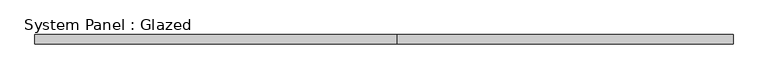
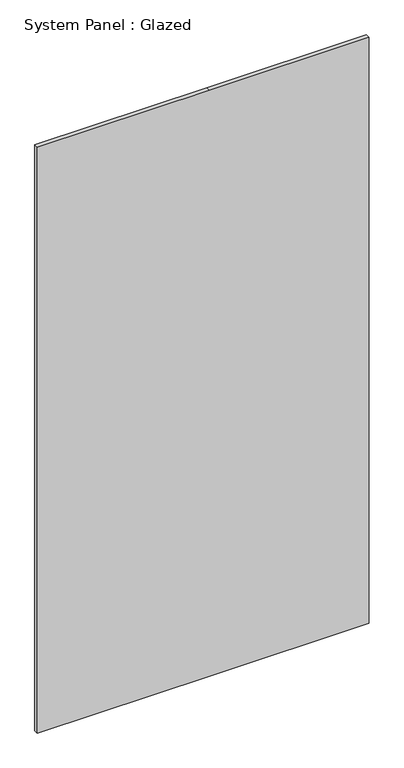
"""IFC4 building model written with IfcOpenShell, lengths in millimetres: plate geometry, System Panel : Glazed."""

import ifcopenshell
import ifcopenshell.guid

model = None  # the IFC model being written
_history = None  # IfcOwnerHistory: only IFC2X3 demands one
_inside = {}  # id of a spatial element -> (the spatial element, [elements in it])
_under = {}  # id of a project, library or spatial element -> (it, [spatial elements below it])
_declared = {}  # id of a project -> (the project, [libraries it declares])
_typed = {}  # id of a type object -> (the type object, [elements of that type])
_made_of = {}  # id of a material, layer set ... -> (it, [elements and type objects made of it])


def new_model(schema):
    """Start an empty IFC model of exactly this schema.

    Asked for "IFC4X3", IfcOpenShell would pick the latest addendum, in which some entities
    have other attributes; the version numbers below select the first issue.
    IFC2X3 requires an IfcOwnerHistory on every rooted entity: one is made here for all.
    """
    global model, _history
    if schema == "IFC4X3":
        model = ifcopenshell.file(schema_version=(4, 3, 0, 0))
    else:
        model = ifcopenshell.file(schema=schema)
    _inside.clear()
    _under.clear()
    _declared.clear()
    _typed.clear()
    _made_of.clear()
    _history = None
    if model.schema == "IFC2X3":
        org = make("IfcOrganization", Name="unknown")
        user = make(
            "IfcPersonAndOrganization",
            ThePerson=make("IfcPerson", FamilyName="unknown"),
            TheOrganization=org,
        )
        app = make(
            "IfcApplication",
            ApplicationDeveloper=org,
            Version="unknown",
            ApplicationFullName="unknown",
            ApplicationIdentifier="unknown",
        )
        _history = make(
            "IfcOwnerHistory",
            OwningUser=user,
            OwningApplication=app,
            ChangeAction="ADDED",
            CreationDate=0,
        )
    return model


def make(cls, **values):
    """One entity of the class cls with the attributes given. An attribute that is None is left unset."""
    return model.create_entity(
        cls, **{name: value for name, value in values.items() if value is not None}
    )


def rooted(cls, **values):
    """An entity with a GlobalId (a new one), such as an element, a storey or a relation."""
    return make(cls, GlobalId=ifcopenshell.guid.new(), OwnerHistory=_history, **values)


def si_unit(unit_type, name, prefix=None):
    """IfcSIUnit, for example si_unit("LENGTHUNIT", "METRE", prefix="MILLI")."""
    return make("IfcSIUnit", UnitType=unit_type, Prefix=prefix, Name=name)


def assignment(units):
    """IfcUnitAssignment: the units of a project."""
    return None if units is None else make("IfcUnitAssignment", Units=units)


def point(xyz):
    """IfcCartesianPoint."""
    return None if xyz is None else make("IfcCartesianPoint", Coordinates=xyz)


def direction(xyz):
    """IfcDirection."""
    return None if xyz is None else make("IfcDirection", DirectionRatios=xyz)


def frame(location, z_axis=None, x_axis=None):
    """IfcAxis2Placement3D, a coordinate frame: its origin and axes. An axis left out is left unset."""
    return make(
        "IfcAxis2Placement3D",
        Location=point(location),
        Axis=direction(z_axis),
        RefDirection=direction(x_axis),
    )


def origin():
    """The frame at (0, 0, 0) with its axes left unset."""
    return frame((0.0, 0.0, 0.0))


def place(relative_to, where):
    """IfcLocalPlacement: puts the frame where relative to a parent placement (None: the world)."""
    return make(
        "IfcLocalPlacement", PlacementRelTo=relative_to, RelativePlacement=where
    )


def context(
    kind, dimensions, precision=None, world=None, true_north=None, identifier=None
):
    """IfcGeometricRepresentationContext, for example the 3D "Model" context."""
    return make(
        "IfcGeometricRepresentationContext",
        ContextIdentifier=identifier,
        ContextType=kind,
        CoordinateSpaceDimension=dimensions,
        Precision=precision,
        WorldCoordinateSystem=world,
        TrueNorth=true_north,
    )


def project(units=None, contexts=None):
    """IfcProject with its units and contexts."""
    return rooted(
        "IfcProject",
        Name="project",
        RepresentationContexts=contexts,
        UnitsInContext=assignment(units),
    )


def spatial(cls, under=None, at=None, **own):
    """A site, building, storey or space (cls), placed at a placement, below another one or the project."""
    s = rooted(cls, ObjectPlacement=at, **own)
    if under is not None:
        _under.setdefault(under.id(), (under, []))[1].append(s)
    return s


def polyline(points):
    """IfcPolyline through the points."""
    return make("IfcPolyline", Points=[point(p) for p in points])


def outline(outer, holes=None, kind="AREA"):
    """IfcArbitraryClosedProfileDef: a profile drawn as a closed curve; with holes, ...WithVoids."""
    if holes is None:
        return make("IfcArbitraryClosedProfileDef", ProfileType=kind, OuterCurve=outer)
    return make(
        "IfcArbitraryProfileDefWithVoids",
        ProfileType=kind,
        OuterCurve=outer,
        InnerCurves=holes,
    )


def extrude(swept, where, along, depth):
    """IfcExtrudedAreaSolid: the profile swept, set in the frame where, extruded along a direction by depth."""
    return make(
        "IfcExtrudedAreaSolid",
        SweptArea=swept,
        Position=where,
        ExtrudedDirection=direction(along),
        Depth=depth,
    )


def shape(context_of_items, identifier, shape_type, items):
    """IfcShapeRepresentation: the items that make up one representation, for example the "Body"."""
    return make(
        "IfcShapeRepresentation",
        ContextOfItems=context_of_items,
        RepresentationIdentifier=identifier,
        RepresentationType=shape_type,
        Items=items,
    )


def source(mapping_origin, context_of_items, identifier, shape_type, items):
    """IfcRepresentationMap: a shape defined once, which mapped items show again and again."""
    return make(
        "IfcRepresentationMap",
        MappingOrigin=mapping_origin,
        MappedRepresentation=shape(context_of_items, identifier, shape_type, items),
    )


def transform(
    local_origin,
    x_axis=None,
    y_axis=None,
    z_axis=None,
    scale=None,
    scale2=None,
    scale3=None,
    uniform=True,
):
    """IfcCartesianTransformationOperator3D, or its non-uniform kind. x_axis, y_axis, z_axis: its Axis1, 2, 3."""
    if uniform:
        return make(
            "IfcCartesianTransformationOperator3D",
            Axis1=direction(x_axis),
            Axis2=direction(y_axis),
            LocalOrigin=point(local_origin),
            Scale=scale,
            Axis3=direction(z_axis),
        )
    return make(
        "IfcCartesianTransformationOperator3DnonUniform",
        Axis1=direction(x_axis),
        Axis2=direction(y_axis),
        LocalOrigin=point(local_origin),
        Scale=scale,
        Axis3=direction(z_axis),
        Scale2=scale2,
        Scale3=scale3,
    )


def mapped(mapping_source, mapping_target):
    """IfcMappedItem: shows the shape of a source again, moved by a transform."""
    return make(
        "IfcMappedItem", MappingSource=mapping_source, MappingTarget=mapping_target
    )


def made_of(thing, what):
    """Note that an element or type object is made of a material, layer set ...; save() writes the relation."""
    if what is not None:
        _made_of.setdefault(what.id(), (what, []))[1].append(thing)
    return thing


def element(
    cls,
    number,
    at=None,
    inside=None,
    cuts=None,
    type_object=None,
    material=None,
    context=None,
    identifier="Body",
    shape_type=None,
    held_by="IfcProductDefinitionShape",
    body=None,
    shapes=None,
    **own,
):
    """One element of the class cls, such as IfcWall. Its Tag is "e" and its number.

    at: its placement. inside: the storey or other place that contains it. cuts: it is an
    opening in that element (IfcRelVoidsElement). A single representation is given by context,
    identifier, shape_type and body (its items); several are given by shapes. held_by: the class
    of the entity that holds the representations. save() writes the other relations.
    """
    e = rooted(cls, Tag="e%d" % number, ObjectPlacement=at, **own)
    if body is not None:
        shapes = [shape(context, identifier, shape_type, body)]
    if shapes is not None:
        e.Representation = make(held_by, Representations=shapes)
    if inside is not None:
        _inside.setdefault(inside.id(), (inside, []))[1].append(e)
    if cuts is not None:
        rooted(
            "IfcRelVoidsElement", RelatingBuildingElement=cuts, RelatedOpeningElement=e
        )
    if type_object is not None:
        _typed.setdefault(type_object.id(), (type_object, []))[1].append(e)
    return made_of(e, material)


def aggregate(whole, parts):
    """IfcRelAggregates: a whole, such as a stair, and the parts it consists of."""
    return rooted("IfcRelAggregates", RelatingObject=whole, RelatedObjects=parts)


def save(model, path):
    """Write the relations noted so far, then the file.

    IfcRelAggregates (storeys below a building ...), IfcRelContainedInSpatialStructure (elements
    in a storey), IfcRelDefinesByType, IfcRelAssociatesMaterial and IfcRelDeclares: one each for
    every whole, place, type object, material and project.
    """
    for whole, parts in _under.values():
        aggregate(whole, parts)
    for where, things in _inside.values():
        rooted(
            "IfcRelContainedInSpatialStructure",
            RelatedElements=things,
            RelatingStructure=where,
        )
    for kind, things in _typed.values():
        rooted("IfcRelDefinesByType", RelatedObjects=things, RelatingType=kind)
    for what, things in _made_of.values():
        rooted("IfcRelAssociatesMaterial", RelatedObjects=things, RelatingMaterial=what)
    for by, libraries in _declared.values():
        rooted("IfcRelDeclares", RelatingContext=by, RelatedDefinitions=libraries)
    model.write(path)


def system_panel_glazed_5e1ca041(model_context):
    return source(origin(), model_context, "Body", "SweptSolid", [
        extrude(outline(polyline([(0.0, -971.55), (0.0, 37.0416667), (0.0, 971.55), (3625.85, 971.55), (3625.85, 37.0416667), (3625.85, -971.55), (0.0, -971.55)])), frame((0.0, -44.45, 0.0), z_axis=(0.0, 1.0, 0.0), x_axis=(0.0, 0.0, 1.0)), (0.0, 0.0, 1.0), 25.4),
    ])


if __name__ == "__main__":
    model = new_model("IFC4")
    model_context = context("Model", 3, world=origin())
    ifc_project = project(units=[si_unit("LENGTHUNIT", "METRE", prefix="MILLI")], contexts=[model_context])
    site = spatial("IfcSite", under=ifc_project)
    building = spatial("IfcBuilding", under=site)
    placement = place(None, origin())
    system_panel_glazed_shape = system_panel_glazed_5e1ca041(model_context)
    element("IfcPlate", 1, ObjectType="System Panel : Glazed", at=placement, inside=building, context=model_context, shape_type="MappedRepresentation", body=[
        mapped(system_panel_glazed_shape, transform((0.0, 0.0, 0.0), x_axis=(1.0, 0.0, 0.0), y_axis=(0.0, 1.0, 0.0), z_axis=(0.0, 0.0, 1.0))),
    ])
    save(model, "model.ifc")

# Revit data of these elements
# Project information
#   SR Document GUID = "b4c0fe6c-219c-4d32-b912-4513e366b333"
# Element 1 (IfcPlate, "System Panel : Glazed")
#   Materials on its faces: "Glass"
# Materials
#   "Glass": class "Unassigned", colour RGB 0 0 255, transparency 0.75
